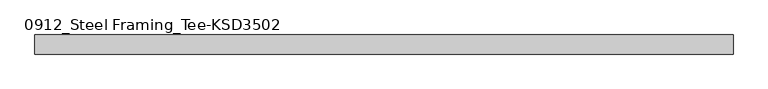
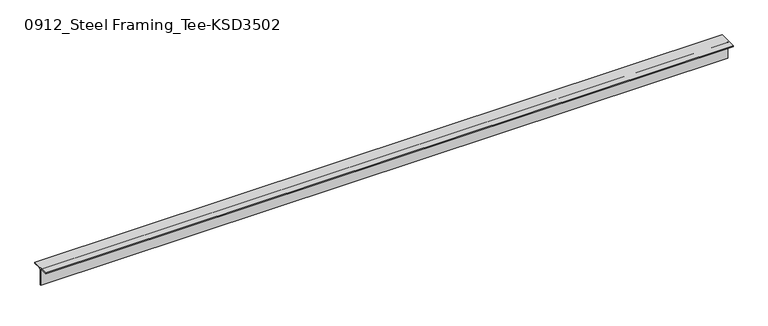
"""IFC4 building model written with IfcOpenShell, lengths in millimetres: member geometry, 0912_Steel Framing_Tee-KSD3502 : H_SB_ASB_CT-150x150x6.5x9."""

from ifc_helpers import new_model, si_unit, point, frame, frame_2d, origin, place, context, project, spatial, polyline, circle_curve, trimmed, segment, composite_curve, outline, extrude, source, transform, mapped, element, save


def member_0912_steel_framing_tee_ksd3502_a607656e(model_context):
    return source(origin(), model_context, "Body", "SweptSolid", [
        extrude(outline(composite_curve([segment(polyline([(-75.0, 75.0), (75.0, 75.0), (75.0, 66.0), (16.25, 66.0)]), True, "CONTINUOUS"), segment(trimmed(circle_curve(frame_2d((16.25, 53.0)), 13.0), [point((16.25, 66.0))], [point((3.25, 53.0))], True, "CARTESIAN"), True, "CONTINUOUS"), segment(polyline([(3.25, 53.0), (3.25, -75.0), (-3.25, -75.0), (-3.25, 53.0)]), True, "CONTINUOUS"), segment(trimmed(circle_curve(frame_2d((-16.25, 53.0)), 13.0), [point((-3.25, 53.0))], [point((-16.25, 66.0))], True, "CARTESIAN"), True, "CONTINUOUS"), segment(polyline([(-16.25, 66.0), (-75.0, 66.0), (-75.0, 75.0)]), True, "CONTINUOUS")], self_intersect=False)), frame((-2725.3, 0.0, 0.0), z_axis=(1.0, 0.0, 0.0), x_axis=(0.0, 1.0, 0.0)), (0.0, 0.0, 1.0), 5477.7),
    ])


if __name__ == "__main__":
    model = new_model("IFC4")
    model_context = context("Model", 3, world=origin())
    ifc_project = project(units=[si_unit("LENGTHUNIT", "METRE", prefix="MILLI")], contexts=[model_context])
    site = spatial("IfcSite", under=ifc_project)
    building = spatial("IfcBuilding", under=site)
    placement = place(None, origin())
    member_0912_steel_framing_tee_ksd3502_shape = member_0912_steel_framing_tee_ksd3502_a607656e(model_context)
    element("IfcMember", 1, ObjectType="0912_Steel Framing_Tee-KSD3502 : H_SB_ASB_CT-150x150x6.5x9", at=placement, inside=building, context=model_context, shape_type="MappedRepresentation", body=[
        mapped(member_0912_steel_framing_tee_ksd3502_shape, transform((0.0, 0.0, 0.0), x_axis=(1.0, 0.0, 0.0), y_axis=(0.0, 1.0, 0.0), z_axis=(0.0, 0.0, 1.0))),
    ])
    save(model, "model.ifc")

# Revit data of these elements
# Type "0912_Steel Framing_Tee-KSD3502 : H_SB_ASB_CT-150x150x6.5x9"
#   H_WM Code_1 = "S01AA003-00001 | Main Steel Structure Fabrication Work | Shelter/Building | Light Steel - Standard (30KG/M>Weight) | Material: (   )"
#   H_WM Code_2 = "S03AA029-00001 | Main Steel Structure Erection Work | Shelter/Building | Light Steel (30KG/M>Weight) | Material: (   )"
#   H_WM Code_3 = "S01AA010-00001 | Main Steel Structure Fabrication Work | Shelter/Building | Steel Painting/Coating | for Non-Fireproofed Steel Surface, Surface Preparation, Primer, Second & Final Coat | Material: (   )"
#   H_Q'ty Cal Type Tag = "SB-Q2"
#   Width = 15.0 cm
#   Web Thickness = 0.65 cm
#   Web Fillet = 1.3 cm
#   Section Area = 23.39 cm²
#   Perimeter = 0.60 m²/m
#   Nominal Weight = 18.40 kgf/m
#   Height = 15.0 cm
#   Flange Thickness = 0.9 cm
#   Centroid Vertical = 7.5 cm
#   Centroid Horizontal = 7.5 cm
#   Length [instance default] = 1.5000 m
#   Structural Material [instance default] = Steel, 45-345
#   Warping Constant = (empty or 0)
#   Torsional Moment of Inertia = 0
#   Section Name Key = ""
#   Plastic Modulus weak axis = 0
#   Plastic Modulus strong axis = 0
#   Moment of Inertia weak axis = 0
#   Moment of Inertia strong axis = 0
#   Elastic Modulus weak axis = 0
#   Elastic Modulus strong axis = 0
#   Bolt Spacing = 0
#   Assembly Code = ""
# Element 1 (IfcMember, "0912_Steel Framing_Tee-KSD3502 : H_SB_ASB_CT-150x150x6.5x9")
#   Structural Material = none
# Materials
#   "Steel, 45-345": class "Metal", colour RGB 189 187 185, transparency 0, Description = "Steel 345 MPa", Cost = 0
